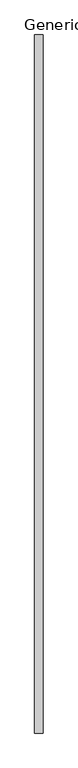
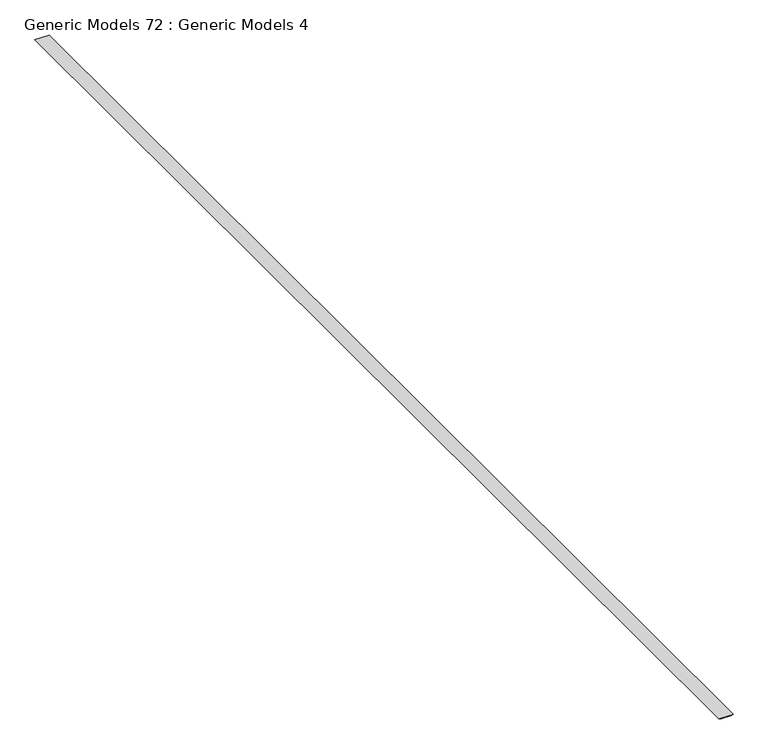
"""IFC4 building model written with IfcOpenShell, lengths in millimetres: proxy geometry, Generic Models 72 : Generic Models 4."""

from ifc_helpers import new_model, si_unit, frame, origin, place, context, project, spatial, polyline, outline, extrude, source, transform, mapped, element, save


def generic_models_72_generic_models_4_992969ca(model_context):
    return source(origin(), model_context, "Body", "SweptSolid", [
        extrude(outline(polyline([(126933.5840478, -8176.334981), (126950.6852144, -8143.0327093), (126955.2896197, -8367.6802697), (126936.7665653, -8331.6090585), (126933.5840478, -8176.334981)])), frame((0.0, -6864.9230338, 0.0), z_axis=(0.0, 1.0, 0.0), x_axis=(0.0, 0.0, 1.0)), (0.0, 0.0, 1.0), 18643.6),
    ])


if __name__ == "__main__":
    model = new_model("IFC4")
    model_context = context("Model", 3, world=origin())
    ifc_project = project(units=[si_unit("LENGTHUNIT", "METRE", prefix="MILLI")], contexts=[model_context])
    site = spatial("IfcSite", under=ifc_project)
    building = spatial("IfcBuilding", under=site)
    placement = place(None, origin())
    generic_models_72_generic_models_4_shape = generic_models_72_generic_models_4_992969ca(model_context)
    element("IfcBuildingElementProxy", 1, Name="Generic Models 72 : Generic Models 4", ObjectType="Generic Models 72 : Generic Models 4", at=placement, inside=building, context=model_context, shape_type="MappedRepresentation", body=[
        mapped(generic_models_72_generic_models_4_shape, transform((0.0, 0.0, 0.0), x_axis=(1.0, 0.0, 0.0), y_axis=(0.0, 1.0, 0.0), z_axis=(0.0, 0.0, 1.0))),
    ])
    save(model, "model.ifc")

# Revit data of these elements
# Element 1 (IfcBuildingElementProxy, "Generic Models 72 : Generic Models 4")
#   Materials on its faces: "_7/8\" SMOOTH TROWEL EXTERIOR STUCCO (COLOR PER OWNER) @ 2% SLOPE"
# Materials
#   "_7/8\" SMOOTH TROWEL EXTERIOR STUCCO (COLOR PER OWNER) @ 2% SLOPE": class "Generic", colour RGB 233 233 233, transparency 0, Cost = 0
